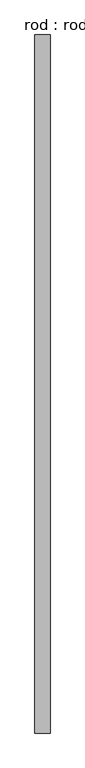
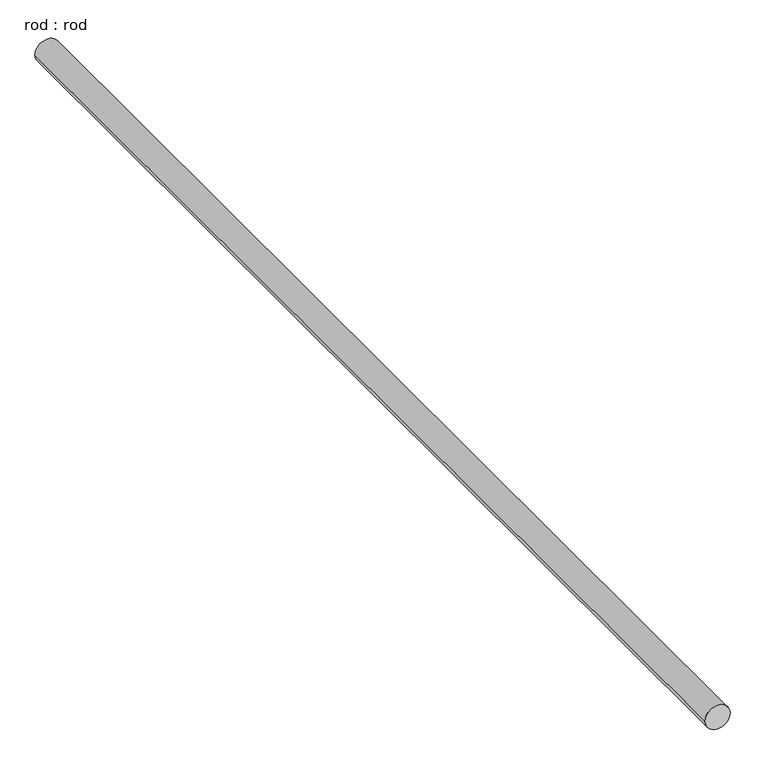
"""IFC4 building model written with IfcOpenShell, lengths in millimetres: proxy geometry, rod : rod."""

from ifc_helpers import new_model, si_unit, point, frame, frame_2d, origin, place, context, project, spatial, circle_curve, trimmed, segment, composite_curve, outline, extrude, source, transform, mapped, element, save


def rod_rod_6de3881e(model_context):
    return source(origin(), model_context, "Body", "SweptSolid", [
        extrude(outline(composite_curve([segment(trimmed(circle_curve(frame_2d((0.0108462, 0.0)), 200.0), [point((0.0108462, 200.0))], [point((0.0108462, -200.0))], False, "CARTESIAN"), True, "CONTINUOUS"), segment(trimmed(circle_curve(frame_2d((0.0108462, 0.0)), 200.0), [point((0.0108462, -200.0))], [point((0.0108462, 200.0))], False, "CARTESIAN"), True, "CONTINUOUS")], self_intersect=False)), frame((0.0, -5157.2713847, 0.0), z_axis=(0.0, 1.0, 0.0), x_axis=(0.0, 0.0, 1.0)), (0.0, 0.0, 1.0), 18500.0),
    ])


if __name__ == "__main__":
    model = new_model("IFC4")
    model_context = context("Model", 3, world=origin())
    ifc_project = project(units=[si_unit("LENGTHUNIT", "METRE", prefix="MILLI")], contexts=[model_context])
    site = spatial("IfcSite", under=ifc_project)
    building = spatial("IfcBuilding", under=site)
    placement = place(None, origin())
    rod_rod_shape = rod_rod_6de3881e(model_context)
    element("IfcBuildingElementProxy", 1, Name="rod : rod", ObjectType="rod : rod", at=placement, inside=building, context=model_context, shape_type="MappedRepresentation", body=[
        mapped(rod_rod_shape, transform((0.0, 0.0, 0.0), x_axis=(1.0, 0.0, 0.0), y_axis=(0.0, 1.0, 0.0), z_axis=(0.0, 0.0, 1.0))),
    ])
    save(model, "model.ifc")

# Revit data of these elements
# Type "rod : rod"
#   Default Elevation = 0
